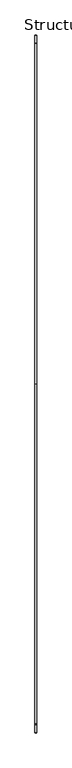
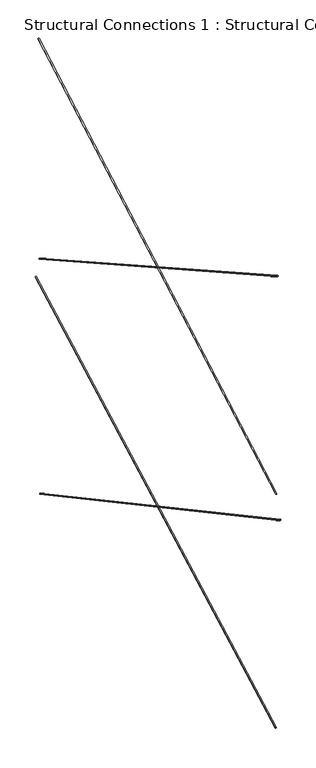
"""IFC4 building model written with IfcOpenShell, lengths in millimetres: fastener geometry, Structural Connections 1 : Structural Connections 1."""

from ifc_helpers import new_model, si_unit, point, frame, frame_2d, origin, place, context, project, spatial, circle_curve, trimmed, segment, composite_curve, outline, extrude, source, transform, mapped, element, save


def structural_connections_1_structural_connections_1_e34a3426(model_context):
    return source(origin(), model_context, "Body", "SweptSolid", [
        extrude(outline(composite_curve([segment(trimmed(circle_curve(frame_2d((0.0, -6.35)), 6.35), [point((0.0, -12.7))], [point((0.0, 0.0))], False, "CARTESIAN"), True, "CONTINUOUS"), segment(trimmed(circle_curve(frame_2d((0.0, -6.35)), 6.35), [point((0.0, 0.0))], [point((0.0, -12.7))], False, "CARTESIAN"), True, "CONTINUOUS")], self_intersect=False)), frame((31983.3710525, 30839.4281612, 266395.2), z_axis=(0.0, 0.8799358799272629, 0.4750924617552184), x_axis=(0.0, -0.4750924617552184, 0.8799358799272629)), (0.0, 0.0, 1.0), 5222.2527547),
        extrude(outline(composite_curve([segment(trimmed(circle_curve(frame_2d((0.0, -6.35)), 6.35), [point((0.0, -12.7))], [point((0.0, 0.0))], False, "CARTESIAN"), True, "CONTINUOUS"), segment(trimmed(circle_curve(frame_2d((0.0, -6.35)), 6.35), [point((0.0, 0.0))], [point((0.0, -12.7))], False, "CARTESIAN"), True, "CONTINUOUS")], self_intersect=False)), frame((31983.3710525, 35348.5582942, 266395.2), z_axis=(0.0, -0.8799358799272629, 0.4750924617552184), x_axis=(0.0, -0.4750924617552184, -0.8799358799272629)), (0.0, 0.0, 1.0), 5222.2527547),
        extrude(outline(composite_curve([segment(trimmed(circle_curve(frame_2d((0.0, -6.35)), 6.35), [point((0.0, -12.7))], [point((0.0, 0.0))], False, "CARTESIAN"), True, "CONTINUOUS"), segment(trimmed(circle_curve(frame_2d((0.0, -6.35)), 6.35), [point((0.0, 0.0))], [point((0.0, -12.7))], False, "CARTESIAN"), True, "CONTINUOUS")], self_intersect=False)), frame((31983.3710525, 35359.7243826, 269132.1193757), z_axis=(0.0, -0.8715855554938525, 0.49024342877235244), x_axis=(0.0, -0.49024342877235244, -0.8715855554938525)), (0.0, 0.0, 1.0), 5222.2527547),
        extrude(outline(composite_curve([segment(trimmed(circle_curve(frame_2d((0.0, -6.35)), 6.35), [point((0.0, -12.7))], [point((0.0, 0.0))], False, "CARTESIAN"), True, "CONTINUOUS"), segment(trimmed(circle_curve(frame_2d((0.0, -6.35)), 6.35), [point((0.0, 0.0))], [point((0.0, -12.7))], False, "CARTESIAN"), True, "CONTINUOUS")], self_intersect=False)), frame((31983.3710525, 30828.2620728, 269132.1193757), z_axis=(0.0, 0.8715855554938525, 0.49024342877235244), x_axis=(0.0, -0.49024342877235244, 0.8715855554938525)), (0.0, 0.0, 1.0), 5222.2527547),
    ])


if __name__ == "__main__":
    model = new_model("IFC4")
    model_context = context("Model", 3, world=origin())
    ifc_project = project(units=[si_unit("LENGTHUNIT", "METRE", prefix="MILLI")], contexts=[model_context])
    site = spatial("IfcSite", under=ifc_project)
    building = spatial("IfcBuilding", under=site)
    placement = place(None, origin())
    structural_connections_1_structural_connections_1_shape = structural_connections_1_structural_connections_1_e34a3426(model_context)
    element("IfcFastener", 1, ObjectType="Structural Connections 1 : Structural Connections 1", at=placement, inside=building, context=model_context, shape_type="MappedRepresentation", body=[
        mapped(structural_connections_1_structural_connections_1_shape, transform((0.0, 0.0, 0.0), x_axis=(1.0, 0.0, 0.0), y_axis=(0.0, 1.0, 0.0), z_axis=(0.0, 0.0, 1.0))),
    ])
    save(model, "model.ifc")
